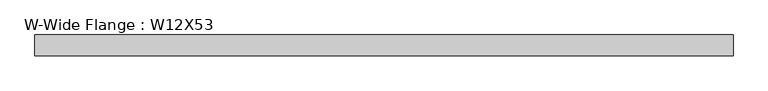
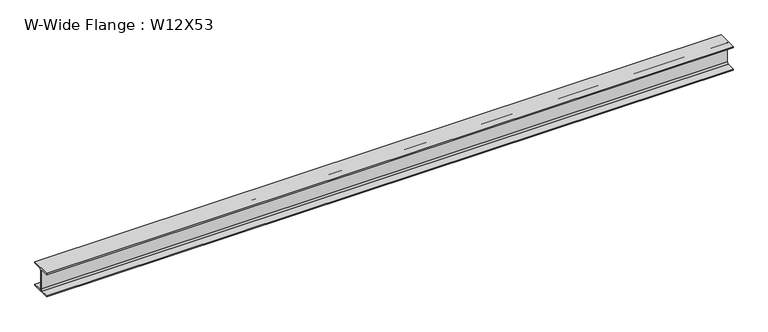
"""IFC4 building model written with IfcOpenShell, lengths in millimetres: beam geometry, W-Wide Flange : W12X53."""

from ifc_helpers import new_model, si_unit, point, frame, frame_2d, origin, place, context, project, spatial, polyline, circle_curve, trimmed, segment, composite_curve, outline, extrude, source, transform, mapped, element, save


def w_wide_flange_w12x53_96ffc1ec(model_context):
    return source(origin(), model_context, "Body", "SweptSolid", [
        extrude(outline(composite_curve([segment(polyline([(127.0, -139.065), (127.0, -153.67), (-127.0, -153.67), (-127.0, -139.065), (-24.7015, -139.065)]), True, "CONTINUOUS"), segment(trimmed(circle_curve(frame_2d((-24.7015, -118.745)), 20.32), [point((-24.7015, -139.065))], [point((-4.3815, -118.745))], True, "CARTESIAN"), True, "CONTINUOUS"), segment(polyline([(-4.3815, -118.745), (-4.3815, 118.745)]), True, "CONTINUOUS"), segment(trimmed(circle_curve(frame_2d((-24.7015, 118.745)), 20.32), [point((-4.3815, 118.745))], [point((-24.7015, 139.065))], True, "CARTESIAN"), True, "CONTINUOUS"), segment(polyline([(-24.7015, 139.065), (-127.0, 139.065), (-127.0, 153.67), (127.0, 153.67), (127.0, 139.065), (24.7015, 139.065)]), True, "CONTINUOUS"), segment(trimmed(circle_curve(frame_2d((24.7015, 118.745)), 20.32), [point((24.7015, 139.065))], [point((4.3815, 118.745))], True, "CARTESIAN"), True, "CONTINUOUS"), segment(polyline([(4.3815, 118.745), (4.3815, -118.745)]), True, "CONTINUOUS"), segment(trimmed(circle_curve(frame_2d((24.7015, -118.745)), 20.32), [point((4.3815, -118.745))], [point((24.7015, -139.065))], True, "CARTESIAN"), True, "CONTINUOUS"), segment(polyline([(24.7015, -139.065), (127.0, -139.065)]), True, "CONTINUOUS")], self_intersect=False)), frame((-4221.9066406, 0.0, 0.0), z_axis=(1.0, 0.0, 0.0), x_axis=(0.0, 1.0, 0.0)), (0.0, 0.0, 1.0), 8493.8195313),
    ])


if __name__ == "__main__":
    model = new_model("IFC4")
    model_context = context("Model", 3, world=origin())
    ifc_project = project(units=[si_unit("LENGTHUNIT", "METRE", prefix="MILLI")], contexts=[model_context])
    site = spatial("IfcSite", under=ifc_project)
    building = spatial("IfcBuilding", under=site)
    placement = place(None, origin())
    w_wide_flange_w12x53_shape = w_wide_flange_w12x53_96ffc1ec(model_context)
    element("IfcBeam", 1, ObjectType="W-Wide Flange : W12X53", at=placement, inside=building, context=model_context, shape_type="MappedRepresentation", body=[
        mapped(w_wide_flange_w12x53_shape, transform((0.0, 0.0, 0.0), x_axis=(1.0, 0.0, 0.0), y_axis=(0.0, 1.0, 0.0), z_axis=(0.0, 0.0, 1.0))),
    ])
    save(model, "model.ifc")

# Revit data of these elements
# Type "W-Wide Flange : W12X53"
#   Assembly Code = "B10"
#   W = 53
#   Length [instance default] = 1524 mm
#   bf = 254 mm
#   d = 307.34 mm
#   k = 34.925 mm
#   k2 = 20.32 mm
#   tf = 14.605 mm
#   tw = 8.763 mm
#   A = 0.0100645 m²
#   Structural Material [instance default] = Steel ASTM A992
# Element 1 (IfcBeam, "W-Wide Flange : W12X53")
#   Structural Material = Aluminum, Anodized Red
#   Materials on its faces: "Aluminum, Anodized Red"
# Materials
#   "Steel ASTM A992": class "Metal", colour RGB 128 0 0, transparency 0, Description = "Structural steel 50ksi", Cost = 0
#   "Aluminum, Anodized Red": class "Metal", colour RGB 120 120 120, transparency 0, Description = "Anodized aluminum, red", Cost = 0
